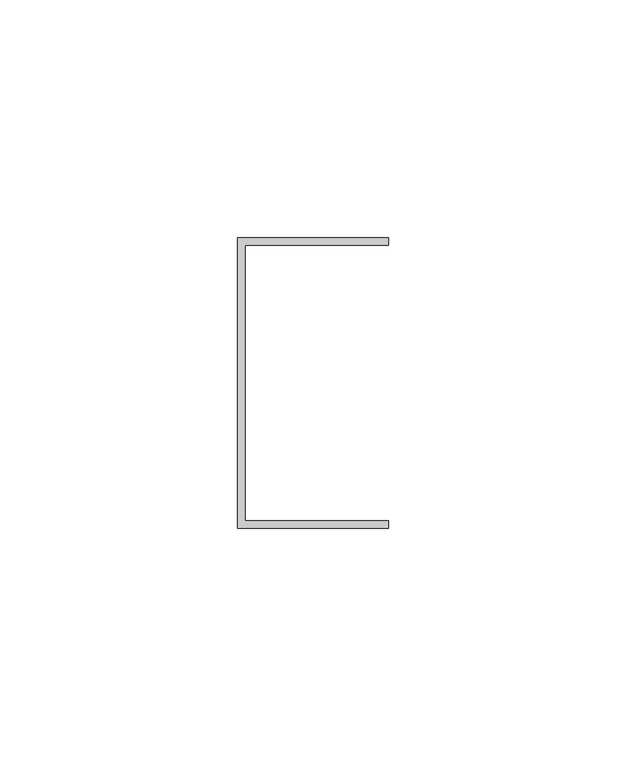
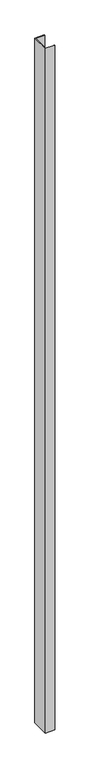
"""IFC4 building model written with IfcOpenShell, lengths in millimetres: proxy geometry, Generic Models 7:Generic Models 1:3:Generic Models 1:3 : Generic Models 7:Generic Models 1:305549:3:Generic Models 1:3:Generic Models 1:3 : Generic Models 7:Generic Models 1:305549:3 : Generic Models 7:Generic Models 1:3:Generic Models 1:3 : Generic Models 7:Generic Models 1:305549:301244:8 : Generic Models 7:Generic Models 1:3:Generic Models 1:3 : Generic Models 7:Generic Models 1:305549:3:Generic Models 1:3:Generic Models 1:3 : Generic Models 7:Generic Models 1:305549:3 : Generic Models 7:Generic Models 1:3:Generic Models 1:3 : Generic Models 7:Generic Models 1:305549:301244:308848."""

from ifc_helpers import new_model, si_unit, frame, origin, place, context, project, spatial, polyline, outline, extrude, source, transform, mapped, element, save


def generic_models_d5db5a45(model_context):
    return source(origin(), model_context, "Body", "SweptSolid", [
        extrude(outline(polyline([(560603.7867239, -579015.772634), (560635.5367239, -579015.772634), (560635.5367239, -579017.360134), (560605.3742239, -579017.360134), (560605.3742239, -579075.303884), (560635.5367239, -579075.303884), (560635.5367239, -579076.891384), (560603.7867239, -579076.891384), (560603.7867239, -579015.772634)])), frame((0.0, 0.0, 3721.1), z_axis=(0.0, 0.0, 1.0), x_axis=(1.0, 0.0, 0.0)), (0.0, 0.0, 1.0), 2430.9324376),
    ])


if __name__ == "__main__":
    model = new_model("IFC4")
    model_context = context("Model", 3, world=origin())
    ifc_project = project(units=[si_unit("LENGTHUNIT", "METRE", prefix="MILLI")], contexts=[model_context])
    site = spatial("IfcSite", under=ifc_project)
    building = spatial("IfcBuilding", under=site)
    placement = place(None, origin())
    generic_models_shape = generic_models_d5db5a45(model_context)
    element("IfcBuildingElementProxy", 1, Name="Generic Models 7:Generic Models 1:3:Generic Models 1:3 : Generic Models 7:Generic Models 1:305549:3:Generic Models 1:3:Generic Models 1:3 : Generic Models 7:Generic Models 1:305549:3 : Generic Models 7:Generic Models 1:3:Generic Models 1:3 : Generic Models 7:Generic Models 1:305549:301244:8 : Generic Models 7:Generic Models 1:3:Generic Models 1:3 : Generic Models 7:Generic Models 1:305549:3:Generic Models 1:3:Generic Models 1:3 : Generic Models 7:Generic Models 1:305549:3 : Generic Models 7:Generic Models 1:3:Generic Models 1:3 : Generic Models 7:Generic Models 1:305549:301244:308848", ObjectType="Generic Models 7:Generic Models 1:3:Generic Models 1:3 : Generic Models 7:Generic Models 1:305549:3:Generic Models 1:3:Generic Models 1:3 : Generic Models 7:Generic Models 1:305549:3 : Generic Models 7:Generic Models 1:3:Generic Models 1:3 : Generic Models 7:Generic Models 1:305549:301244:8 : Generic Models 7:Generic Models 1:3:Generic Models 1:3 : Generic Models 7:Generic Models 1:305549:3:Generic Models 1:3:Generic Models 1:3 : Generic Models 7:Generic Models 1:305549:3 : Generic Models 7:Generic Models 1:3:Generic Models 1:3 : Generic Models 7:Generic Models 1:305549:301244:308848", at=placement, inside=building, context=model_context, shape_type="MappedRepresentation", body=[
        mapped(generic_models_shape, transform((0.0, 0.0, 0.0), x_axis=(1.0, 0.0, 0.0), y_axis=(0.0, 1.0, 0.0), z_axis=(0.0, 0.0, 1.0))),
    ])
    save(model, "model.ifc")

# Revit data of these elements
# Type "Generic Models 7:Generic Models 1:3:Generic Models 1:3 : Generic Models 7:Generic Models 1:305549:3:Generic Models 1:3:Generic Models 1:3 : Generic Models 7:Generic Models 1:305549:3 : Generic Models 7:Generic Models 1:3:Generic Models 1:3 : Generic Models 7:Generic Models 1:305549:301244:8 : Generic Models 7:Generic Models 1:3:Generic Models 1:3 : Generic Models 7:Generic Models 1:305549:3:Generic Models 1:3:Generic Models 1:3 : Generic Models 7:Generic Models 1:305549:3 : Generic Models 7:Generic Models 1:3:Generic Models 1:3 : Generic Models 7:Generic Models 1:305549:301244:308848"
#   NameOverride = "Generic Models 7:Generic Models 1:3:Generic Models 1:3 : Generic Models 7:Generic Models 1:305549:3:Generic Models 1:3:Generic Models 1:3 : Generic Models 7:Generic Models 1:305549:3 : Generic Models 7:Generic Models 1:3:Generic Models 1:3 : Generic Models 7:Generic Models 1:305549:301244:308848"
#   ObjectTypeOverride = "Generic Models 1:3:Generic Models 1:3 : Generic Models 7:Generic Models 1:305549:3 : Generic Models 7:Generic Models 1:3:Generic Models 1:3 : Generic Models 7:Generic Models 1:305549:301244"
#   Reference = "Generic Models 1"
#   Tag = "308848"
# Element 1 (IfcBuildingElementProxy, "Generic Models 7:Generic Models 1:3:Generic Models 1:3 : Generic Models 7:Generic Models 1:305549:3:Generic Models 1:3:Generic Models 1:3 : Generic Models 7:Generic Models 1:305549:3 : Generic Models 7:Generic Models 1:3:Generic Models 1:3 : Generic Models 7:Generic Models 1:305549:301244:8 : Generic Models 7:Generic Models 1:3:Generic Models 1:3 : Generic Models 7:Generic Models 1:305549:3:Generic Models 1:3:Generic Models 1:3 : Generic Models 7:Generic Models 1:305549:3 : Generic Models 7:Generic Models 1:3:Generic Models 1:3 : Generic Models 7:Generic Models 1:305549:301244:308848")
#   Materials on its faces: "GALVANIZED U-CHANNEL (250T125-33)"
# Materials
#   "GALVANIZED U-CHANNEL (250T125-33)": class "Unassigned", colour RGB 202 201 200, transparency 0, Keynote = "M05451300.02", Cost = 0
